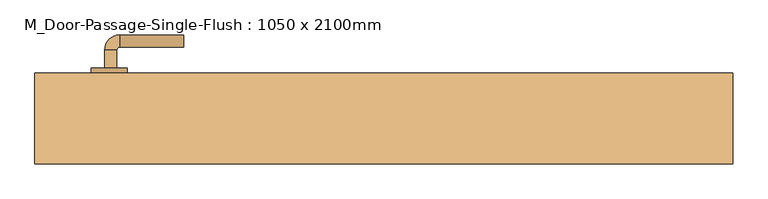
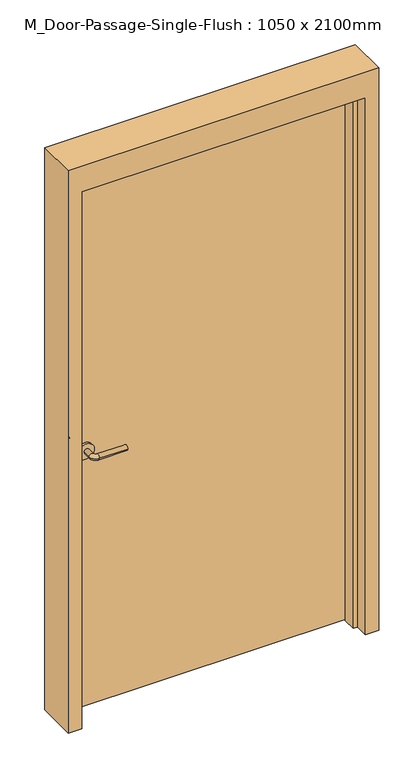
"""IFC4 building model written with IfcOpenShell, lengths in millimetres: door geometry, M_Door-Passage-Single-Flush : 1050 x 2100mm."""

import ifcopenshell
import ifcopenshell.guid

model = None  # the IFC model being written
_history = None  # IfcOwnerHistory: only IFC2X3 demands one
_inside = {}  # id of a spatial element -> (the spatial element, [elements in it])
_under = {}  # id of a project, library or spatial element -> (it, [spatial elements below it])
_declared = {}  # id of a project -> (the project, [libraries it declares])
_typed = {}  # id of a type object -> (the type object, [elements of that type])
_made_of = {}  # id of a material, layer set ... -> (it, [elements and type objects made of it])


def new_model(schema):
    """Start an empty IFC model of exactly this schema.

    Asked for "IFC4X3", IfcOpenShell would pick the latest addendum, in which some entities
    have other attributes; the version numbers below select the first issue.
    IFC2X3 requires an IfcOwnerHistory on every rooted entity: one is made here for all.
    """
    global model, _history
    if schema == "IFC4X3":
        model = ifcopenshell.file(schema_version=(4, 3, 0, 0))
    else:
        model = ifcopenshell.file(schema=schema)
    _inside.clear()
    _under.clear()
    _declared.clear()
    _typed.clear()
    _made_of.clear()
    _history = None
    if model.schema == "IFC2X3":
        org = make("IfcOrganization", Name="unknown")
        user = make(
            "IfcPersonAndOrganization",
            ThePerson=make("IfcPerson", FamilyName="unknown"),
            TheOrganization=org,
        )
        app = make(
            "IfcApplication",
            ApplicationDeveloper=org,
            Version="unknown",
            ApplicationFullName="unknown",
            ApplicationIdentifier="unknown",
        )
        _history = make(
            "IfcOwnerHistory",
            OwningUser=user,
            OwningApplication=app,
            ChangeAction="ADDED",
            CreationDate=0,
        )
    return model


def make(cls, **values):
    """One entity of the class cls with the attributes given. An attribute that is None is left unset."""
    return model.create_entity(
        cls, **{name: value for name, value in values.items() if value is not None}
    )


def rooted(cls, **values):
    """An entity with a GlobalId (a new one), such as an element, a storey or a relation."""
    return make(cls, GlobalId=ifcopenshell.guid.new(), OwnerHistory=_history, **values)


def si_unit(unit_type, name, prefix=None):
    """IfcSIUnit, for example si_unit("LENGTHUNIT", "METRE", prefix="MILLI")."""
    return make("IfcSIUnit", UnitType=unit_type, Prefix=prefix, Name=name)


def assignment(units):
    """IfcUnitAssignment: the units of a project."""
    return None if units is None else make("IfcUnitAssignment", Units=units)


def point(xyz):
    """IfcCartesianPoint."""
    return None if xyz is None else make("IfcCartesianPoint", Coordinates=xyz)


def direction(xyz):
    """IfcDirection."""
    return None if xyz is None else make("IfcDirection", DirectionRatios=xyz)


def frame(location, z_axis=None, x_axis=None):
    """IfcAxis2Placement3D, a coordinate frame: its origin and axes. An axis left out is left unset."""
    return make(
        "IfcAxis2Placement3D",
        Location=point(location),
        Axis=direction(z_axis),
        RefDirection=direction(x_axis),
    )


def frame_2d(location, x_axis=None):
    """IfcAxis2Placement2D, a coordinate frame in the plane: its origin and x axis."""
    return make(
        "IfcAxis2Placement2D", Location=point(location), RefDirection=direction(x_axis)
    )


def origin():
    """The frame at (0, 0, 0) with its axes left unset."""
    return frame((0.0, 0.0, 0.0))


def origin_with_axes():
    """The frame at (0, 0, 0) with the z axis (0, 0, 1) and the x axis (1, 0, 0) written out."""
    return frame((0.0, 0.0, 0.0), z_axis=(0.0, 0.0, 1.0), x_axis=(1.0, 0.0, 0.0))


def place(relative_to, where):
    """IfcLocalPlacement: puts the frame where relative to a parent placement (None: the world)."""
    return make(
        "IfcLocalPlacement", PlacementRelTo=relative_to, RelativePlacement=where
    )


def context(
    kind, dimensions, precision=None, world=None, true_north=None, identifier=None
):
    """IfcGeometricRepresentationContext, for example the 3D "Model" context."""
    return make(
        "IfcGeometricRepresentationContext",
        ContextIdentifier=identifier,
        ContextType=kind,
        CoordinateSpaceDimension=dimensions,
        Precision=precision,
        WorldCoordinateSystem=world,
        TrueNorth=true_north,
    )


def project(units=None, contexts=None):
    """IfcProject with its units and contexts."""
    return rooted(
        "IfcProject",
        Name="project",
        RepresentationContexts=contexts,
        UnitsInContext=assignment(units),
    )


def spatial(cls, under=None, at=None, **own):
    """A site, building, storey or space (cls), placed at a placement, below another one or the project."""
    s = rooted(cls, ObjectPlacement=at, **own)
    if under is not None:
        _under.setdefault(under.id(), (under, []))[1].append(s)
    return s


def polyline(points):
    """IfcPolyline through the points."""
    return make("IfcPolyline", Points=[point(p) for p in points])


def circle_curve(where, radius):
    """IfcCircle in the frame where."""
    return make("IfcCircle", Position=where, Radius=radius)


def ellipse_curve(where, semi_axis1, semi_axis2):
    """IfcEllipse in the frame where."""
    return make(
        "IfcEllipse", Position=where, SemiAxis1=semi_axis1, SemiAxis2=semi_axis2
    )


def trimmed(basis, trim1, trim2, sense, master):
    """IfcTrimmedCurve: the piece of a basis curve between two trims."""
    return make(
        "IfcTrimmedCurve",
        BasisCurve=basis,
        Trim1=trim1,
        Trim2=trim2,
        SenseAgreement=sense,
        MasterRepresentation=master,
    )


def segment(curve, same_sense, transition):
    """IfcCompositeCurveSegment."""
    return make(
        "IfcCompositeCurveSegment",
        Transition=transition,
        SameSense=same_sense,
        ParentCurve=curve,
    )


def composite_curve(segments, self_intersect=None):
    """IfcCompositeCurve: segments joined end to end."""
    return make("IfcCompositeCurve", Segments=segments, SelfIntersect=self_intersect)


def outline(outer, holes=None, kind="AREA"):
    """IfcArbitraryClosedProfileDef: a profile drawn as a closed curve; with holes, ...WithVoids."""
    if holes is None:
        return make("IfcArbitraryClosedProfileDef", ProfileType=kind, OuterCurve=outer)
    return make(
        "IfcArbitraryProfileDefWithVoids",
        ProfileType=kind,
        OuterCurve=outer,
        InnerCurves=holes,
    )


def extrude(swept, where, along, depth):
    """IfcExtrudedAreaSolid: the profile swept, set in the frame where, extruded along a direction by depth."""
    return make(
        "IfcExtrudedAreaSolid",
        SweptArea=swept,
        Position=where,
        ExtrudedDirection=direction(along),
        Depth=depth,
    )


def faces_of(points, faces, orient=None, outer=None):
    """IfcFace entities. A face is a list of loops; a loop is a list of indices into points, from 0.

    orient and outer hold one flag for each loop. By default every Orientation is true, the
    first loop of a face is its IfcFaceOuterBound and the others are IfcFaceBound.
    """
    made = []
    for i, loops in enumerate(faces):
        bounds = []
        for j, loop in enumerate(loops):
            is_outer = j == 0 if outer is None else outer[i][j]
            bounds.append(
                make(
                    "IfcFaceOuterBound" if is_outer else "IfcFaceBound",
                    Bound=make("IfcPolyLoop", Polygon=[points[k] for k in loop]),
                    Orientation=True if orient is None else orient[i][j],
                )
            )
        made.append(make("IfcFace", Bounds=bounds))
    return made


def faceted_brep(points, faces, orient=None, outer=None, voids=None):
    """IfcFacetedBrep: a solid bounded by flat faces; with voids (closed shells), ...WithVoids."""
    shared = [point(p) for p in points]
    hull = make("IfcClosedShell", CfsFaces=faces_of(shared, faces, orient, outer))
    if voids is None:
        return make("IfcFacetedBrep", Outer=hull)
    return make(
        "IfcFacetedBrepWithVoids",
        Outer=hull,
        Voids=[
            make(cls, CfsFaces=faces_of(shared, fs, o, b)) for cls, fs, o, b in voids
        ],
    )


def shape(context_of_items, identifier, shape_type, items):
    """IfcShapeRepresentation: the items that make up one representation, for example the "Body"."""
    return make(
        "IfcShapeRepresentation",
        ContextOfItems=context_of_items,
        RepresentationIdentifier=identifier,
        RepresentationType=shape_type,
        Items=items,
    )


def source(mapping_origin, context_of_items, identifier, shape_type, items):
    """IfcRepresentationMap: a shape defined once, which mapped items show again and again."""
    return make(
        "IfcRepresentationMap",
        MappingOrigin=mapping_origin,
        MappedRepresentation=shape(context_of_items, identifier, shape_type, items),
    )


def transform(
    local_origin,
    x_axis=None,
    y_axis=None,
    z_axis=None,
    scale=None,
    scale2=None,
    scale3=None,
    uniform=True,
):
    """IfcCartesianTransformationOperator3D, or its non-uniform kind. x_axis, y_axis, z_axis: its Axis1, 2, 3."""
    if uniform:
        return make(
            "IfcCartesianTransformationOperator3D",
            Axis1=direction(x_axis),
            Axis2=direction(y_axis),
            LocalOrigin=point(local_origin),
            Scale=scale,
            Axis3=direction(z_axis),
        )
    return make(
        "IfcCartesianTransformationOperator3DnonUniform",
        Axis1=direction(x_axis),
        Axis2=direction(y_axis),
        LocalOrigin=point(local_origin),
        Scale=scale,
        Axis3=direction(z_axis),
        Scale2=scale2,
        Scale3=scale3,
    )


def mapped(mapping_source, mapping_target):
    """IfcMappedItem: shows the shape of a source again, moved by a transform."""
    return make(
        "IfcMappedItem", MappingSource=mapping_source, MappingTarget=mapping_target
    )


def made_of(thing, what):
    """Note that an element or type object is made of a material, layer set ...; save() writes the relation."""
    if what is not None:
        _made_of.setdefault(what.id(), (what, []))[1].append(thing)
    return thing


def element(
    cls,
    number,
    at=None,
    inside=None,
    cuts=None,
    type_object=None,
    material=None,
    context=None,
    identifier="Body",
    shape_type=None,
    held_by="IfcProductDefinitionShape",
    body=None,
    shapes=None,
    **own,
):
    """One element of the class cls, such as IfcWall. Its Tag is "e" and its number.

    at: its placement. inside: the storey or other place that contains it. cuts: it is an
    opening in that element (IfcRelVoidsElement). A single representation is given by context,
    identifier, shape_type and body (its items); several are given by shapes. held_by: the class
    of the entity that holds the representations. save() writes the other relations.
    """
    e = rooted(cls, Tag="e%d" % number, ObjectPlacement=at, **own)
    if body is not None:
        shapes = [shape(context, identifier, shape_type, body)]
    if shapes is not None:
        e.Representation = make(held_by, Representations=shapes)
    if inside is not None:
        _inside.setdefault(inside.id(), (inside, []))[1].append(e)
    if cuts is not None:
        rooted(
            "IfcRelVoidsElement", RelatingBuildingElement=cuts, RelatedOpeningElement=e
        )
    if type_object is not None:
        _typed.setdefault(type_object.id(), (type_object, []))[1].append(e)
    return made_of(e, material)


def aggregate(whole, parts):
    """IfcRelAggregates: a whole, such as a stair, and the parts it consists of."""
    return rooted("IfcRelAggregates", RelatingObject=whole, RelatedObjects=parts)


def save(model, path):
    """Write the relations noted so far, then the file.

    IfcRelAggregates (storeys below a building ...), IfcRelContainedInSpatialStructure (elements
    in a storey), IfcRelDefinesByType, IfcRelAssociatesMaterial and IfcRelDeclares: one each for
    every whole, place, type object, material and project.
    """
    for whole, parts in _under.values():
        aggregate(whole, parts)
    for where, things in _inside.values():
        rooted(
            "IfcRelContainedInSpatialStructure",
            RelatedElements=things,
            RelatingStructure=where,
        )
    for kind, things in _typed.values():
        rooted("IfcRelDefinesByType", RelatedObjects=things, RelatingType=kind)
    for what, things in _made_of.values():
        rooted("IfcRelAssociatesMaterial", RelatedObjects=things, RelatingMaterial=what)
    for by, libraries in _declared.values():
        rooted("IfcRelDeclares", RelatingContext=by, RelatedDefinitions=libraries)
    model.write(path)


def plane_surface(at):
    """IfcPlane: the flat surface through the origin of the frame at, square to its z axis."""
    return make("IfcPlane", Position=at)


def cylinder_surface(at, radius):
    """IfcCylindricalSurface: all points at the distance radius from the z axis of the frame at."""
    return make("IfcCylindricalSurface", Position=at, Radius=radius)


def revolved_surface(curve, axis_point, axis_direction):
    """IfcSurfaceOfRevolution: the curve turned about the line through axis_point along axis_direction."""
    return make(
        "IfcSurfaceOfRevolution",
        SweptCurve=make("IfcArbitraryOpenProfileDef", ProfileType="CURVE", Curve=curve),
        AxisPosition=make("IfcAxis1Placement", Location=point(axis_point), Axis=direction(axis_direction)),
    )


def advanced_brep(points, edges, surfaces, faces):
    """IfcAdvancedBrep: a solid bounded by faces that lie on surfaces and meet in shared edges.

    An edge is (start, end): straight between two places in points (the first is 0);
    or (start, end, curve); or (start, end, curve, False) where it runs against its curve.
    A face is (place in surfaces, loops), or (place, loops, False) where it looks against
    its surface's normal. A loop lists edges by number (the first is 1), with a minus sign
    where the edge is run from its end to its start. The first loop is the outer one.
    """
    corners = [point(p) for p in points]
    vertices = [make("IfcVertexPoint", VertexGeometry=c) for c in corners]
    made = []
    for start, end, *more in edges:
        made.append(
            make(
                "IfcEdgeCurve",
                EdgeStart=vertices[start],
                EdgeEnd=vertices[end],
                EdgeGeometry=more[0] if more else make("IfcPolyline", Points=[corners[start], corners[end]]),
                SameSense=more[1] if len(more) > 1 else True,
            )
        )
    hull = []
    for where, loops, *sense in faces:
        bounds = []
        for j, loop in enumerate(loops):
            ring = [make("IfcOrientedEdge", EdgeElement=made[abs(k) - 1], Orientation=k > 0) for k in loop]
            bounds.append(
                make(
                    "IfcFaceOuterBound" if j == 0 else "IfcFaceBound",
                    Bound=make("IfcEdgeLoop", EdgeList=ring),
                    Orientation=True,
                )
            )
        hull.append(make("IfcAdvancedFace", Bounds=bounds, FaceSurface=surfaces[where], SameSense=sense[0] if sense else True))
    return make("IfcAdvancedBrep", Outer=make("IfcClosedShell", CfsFaces=hull))


def m_door_passage_single_flush_1050_x_2100mm_780507da(model_context):
    return source(origin(), model_context, "Body", "SolidModel", [
        advanced_brep(
        [(-459.990625, 78.35, 1000.0), (-439.990625, 78.35, 1000.0), (-439.990625, 48.35, 1000.0), (-459.990625, 48.35, 1000.0), (-434.990625, 43.35, 1000.0), (-434.990625, 23.35, 1000.0), (-329.990625, 23.35, 1000.0), (-329.990625, 43.35, 1000.0)],
        [
            (0, 1, circle_curve(frame((-449.990625, 78.35, 1000.0), z_axis=(0.0, 1.0, 0.0), x_axis=(1.0, 0.0, 0.0)), 10.0)),
            (1, 0, circle_curve(frame((-449.990625, 78.35, 1000.0), z_axis=(0.0, 1.0, 0.0), x_axis=(1.0, 0.0, 0.0)), 10.0)),
            (1, 2),
            (2, 3, circle_curve(frame((-449.990625, 48.35, 1000.0), z_axis=(0.0, 1.0, 0.0), x_axis=(1.0, 0.0, 0.0)), 10.0)),
            (3, 0),
            (3, 2, circle_curve(frame((-449.990625, 48.35, 1000.0), z_axis=(0.0, 1.0, 0.0), x_axis=(1.0, 0.0, 0.0)), 10.0)),
            (4, 5, circle_curve(frame((-434.990625, 33.35, 1000.0), z_axis=(-1.0, 0.0, 0.0), x_axis=(0.0, 1.0, 0.0)), 10.0)),
            (5, 3, circle_curve(frame((-434.990625, 48.35, 1000.0), z_axis=(0.0, 0.0, -1.0), x_axis=(-1.0, 0.0, 0.0)), 25.0)),
            (2, 4, circle_curve(frame((-434.990625, 48.35, 1000.0), z_axis=(0.0, 0.0, 1.0), x_axis=(-1.0, 0.0, 0.0)), 5.0)),
            (5, 4, circle_curve(frame((-434.990625, 33.35, 1000.0), z_axis=(-1.0, 0.0, 0.0), x_axis=(0.0, 1.0, 0.0)), 10.0)),
            (6, 7, circle_curve(frame((-329.990625, 33.35, 1000.0), z_axis=(1.0, 0.0, 0.0), x_axis=(0.0, 1.0, 0.0)), 10.0)),
            (7, 6, circle_curve(frame((-329.990625, 33.35, 1000.0), z_axis=(1.0, 0.0, 0.0), x_axis=(0.0, 1.0, 0.0)), 10.0)),
            (4, 7),
            (6, 5),
        ],
        [
            plane_surface(frame((-449.990625, 78.35, 1000.0), z_axis=(0.0, 1.0, 0.0), x_axis=(0.0, 0.0, 1.0))),
            cylinder_surface(frame((-449.990625, 78.35, 1000.0), z_axis=(0.0, 1.0, 0.0), x_axis=(1.0, 0.0, 0.0)), 10.0),
            revolved_surface(trimmed(ellipse_curve(frame((-449.990625, 48.35, 1000.0), z_axis=(0.0, -1.0, 0.0), x_axis=(1.0, 0.0, 0.0)), 10.0, 10.0), [point((-459.990625, 48.35, 1000.0))], [point((-439.990625, 48.35, 1000.0))], True, "CARTESIAN"), (-434.990625, 48.35, 1000.0), (0.0, 0.0, -1.0)),
            revolved_surface(trimmed(ellipse_curve(frame((-449.990625, 48.35, 1000.0), z_axis=(0.0, -1.0, 0.0), x_axis=(1.0, 0.0, 0.0)), 10.0, 10.0), [point((-439.990625, 48.35, 1000.0))], [point((-459.990625, 48.35, 1000.0))], True, "CARTESIAN"), (-434.990625, 48.35, 1000.0), (0.0, 0.0, -1.0)),
            plane_surface(frame((-329.990625, 33.35, 1000.0), z_axis=(1.0, 0.0, 0.0), x_axis=(0.0, 0.0, 1.0))),
            cylinder_surface(frame((-434.990625, 33.35, 1000.0), z_axis=(-1.0, 0.0, 0.0), x_axis=(0.0, 1.0, 0.0)), 10.0),
        ],
        [
            (0, [[1, 2]]),
            (1, [[3, 4, 5, -2]]),
            (1, [[-5, 6, -3, -1]]),
            (2, [[7, 8, -4, 9]]),
            (3, [[10, -9, -6, -8]]),
            (4, [[11, 12]]),
            (5, [[13, -11, 14, -7]]),
            (5, [[-14, -12, -13, -10]]),
        ],
    ),
        extrude(outline(composite_curve([segment(trimmed(circle_curve(frame_2d((1000.0, -452.490625)), 30.0), [point((1000.0, -482.490625))], [point((1000.0, -422.490625))], False, "CARTESIAN"), True, "CONTINUOUS"), segment(trimmed(circle_curve(frame_2d((1000.0, -452.490625)), 30.0), [point((1000.0, -422.490625))], [point((1000.0, -482.490625))], False, "CARTESIAN"), True, "CONTINUOUS")], self_intersect=False)), frame((0.0, 78.35, 0.0), z_axis=(0.0, 1.0, 0.0), x_axis=(0.0, 0.0, 1.0)), (0.0, 0.0, 1.0), 8.0),
        advanced_brep(
        [(-459.990625, 139.35, 1000.0), (-439.990625, 139.35, 1000.0), (-459.990625, 169.35, 1000.0), (-439.990625, 169.35, 1000.0), (-434.990625, 174.35, 1000.0), (-434.990625, 194.35, 1000.0), (-329.990625, 194.35, 1000.0), (-329.990625, 174.35, 1000.0)],
        [
            (0, 1, circle_curve(frame((-449.990625, 139.35, 1000.0), z_axis=(0.0, -1.0, 0.0), x_axis=(1.0, 0.0, 0.0)), 10.0)),
            (1, 0, circle_curve(frame((-449.990625, 139.35, 1000.0), z_axis=(0.0, -1.0, 0.0), x_axis=(1.0, 0.0, 0.0)), 10.0)),
            (0, 2),
            (2, 3, circle_curve(frame((-449.990625, 169.35, 1000.0), z_axis=(0.0, -1.0, 0.0), x_axis=(1.0, 0.0, 0.0)), 10.0)),
            (3, 1),
            (3, 2, circle_curve(frame((-449.990625, 169.35, 1000.0), z_axis=(0.0, -1.0, 0.0), x_axis=(1.0, 0.0, 0.0)), 10.0)),
            (4, 3, circle_curve(frame((-434.990625, 169.35, 1000.0), z_axis=(0.0, 0.0, 1.0), x_axis=(-1.0, 0.0, 0.0)), 5.0)),
            (2, 5, circle_curve(frame((-434.990625, 169.35, 1000.0), z_axis=(0.0, 0.0, -1.0), x_axis=(-1.0, 0.0, 0.0)), 25.0)),
            (5, 4, circle_curve(frame((-434.990625, 184.35, 1000.0), z_axis=(-1.0, 0.0, 0.0), x_axis=(0.0, -1.0, 0.0)), 10.0)),
            (4, 5, circle_curve(frame((-434.990625, 184.35, 1000.0), z_axis=(-1.0, 0.0, 0.0), x_axis=(0.0, -1.0, 0.0)), 10.0)),
            (6, 7, circle_curve(frame((-329.990625, 184.35, 1000.0), z_axis=(1.0, 0.0, 0.0), x_axis=(0.0, -1.0, 0.0)), 10.0)),
            (7, 6, circle_curve(frame((-329.990625, 184.35, 1000.0), z_axis=(1.0, 0.0, 0.0), x_axis=(0.0, -1.0, 0.0)), 10.0)),
            (5, 6),
            (7, 4),
        ],
        [
            plane_surface(frame((-449.990625, 139.35, 1000.0), z_axis=(0.0, -1.0, 0.0), x_axis=(0.0, 0.0, 1.0))),
            cylinder_surface(frame((-449.990625, 139.35, 1000.0), z_axis=(0.0, -1.0, 0.0), x_axis=(1.0, 0.0, 0.0)), 10.0),
            revolved_surface(trimmed(ellipse_curve(frame((-449.990625, 169.35, 1000.0), z_axis=(0.0, -1.0, 0.0), x_axis=(1.0, 0.0, 0.0)), 10.0, 10.0), [point((-459.990625, 169.35, 1000.0))], [point((-439.990625, 169.35, 1000.0))], True, "CARTESIAN"), (-434.990625, 169.35, 1000.0), (0.0, 0.0, -1.0)),
            revolved_surface(trimmed(ellipse_curve(frame((-449.990625, 169.35, 1000.0), z_axis=(0.0, -1.0, 0.0), x_axis=(1.0, 0.0, 0.0)), 10.0, 10.0), [point((-439.990625, 169.35, 1000.0))], [point((-459.990625, 169.35, 1000.0))], True, "CARTESIAN"), (-434.990625, 169.35, 1000.0), (0.0, 0.0, -1.0)),
            plane_surface(frame((-329.990625, 184.35, 1000.0), z_axis=(1.0, 0.0, 0.0), x_axis=(0.0, 0.0, 1.0))),
            cylinder_surface(frame((-434.990625, 184.35, 1000.0), z_axis=(-1.0, 0.0, 0.0), x_axis=(0.0, -1.0, 0.0)), 10.0),
        ],
        [
            (0, [[1, 2]]),
            (1, [[-1, 3, 4, 5]]),
            (1, [[-2, -5, 6, -3]]),
            (2, [[7, -4, 8, 9]]),
            (3, [[-8, -6, -7, 10]]),
            (4, [[11, 12]]),
            (5, [[-9, 13, -12, 14]]),
            (5, [[-10, -14, -11, -13]]),
        ],
    ),
        extrude(outline(composite_curve([segment(trimmed(circle_curve(frame_2d((1000.0, -452.490625)), 30.0), [point((1000.0, -482.490625))], [point((1000.0, -422.490625))], False, "CARTESIAN"), True, "CONTINUOUS"), segment(trimmed(circle_curve(frame_2d((1000.0, -452.490625)), 30.0), [point((1000.0, -422.490625))], [point((1000.0, -482.490625))], False, "CARTESIAN"), True, "CONTINUOUS")], self_intersect=False)), frame((0.0, 131.35, 0.0), z_axis=(0.0, 1.0, 0.0), x_axis=(0.0, 0.0, 1.0)), (0.0, 0.0, 1.0), 8.0),
        faceted_brep([(525.0, 81.5875, 0.0), (525.0, 131.35, 0.0), (575.0, 131.35, 0.0), (575.0, -18.65, 0.0), (525.0, -18.65, 0.0), (525.0, 30.5625, 0.0), (509.125, 30.5625, 0.0), (509.125, 81.5875, 0.0), (525.0, 81.5875, 2100.0), (525.0, 131.35, 2100.0), (-525.0, 131.35, 2100.0), (-525.0, 131.35, 0.0), (-575.0, 131.35, 0.0), (-575.0, 131.35, 2200.0), (575.0, 131.35, 2200.0), (575.0, -18.65, 2200.0), (-575.0, -18.65, 2200.0), (-575.0, -18.65, 0.0), (-525.0, -18.65, 0.0), (-525.0, -18.65, 2100.0), (525.0, -18.65, 2100.0), (525.0, 30.5625, 2100.0), (-525.0, 30.5625, 2100.0), (-525.0, 30.5625, 0.0), (-509.125, 30.5625, 0.0), (-509.125, 30.5625, 2084.125), (509.125, 30.5625, 2084.125), (509.125, 81.5875, 2084.125), (-509.125, 81.5875, 2084.125), (-509.125, 81.5875, 0.0), (-525.0, 81.5875, 0.0), (-525.0, 81.5875, 2100.0)], [[[0, 1, 2, 3, 4, 5, 6, 7]], [[1, 0, 8, 9]], [[2, 1, 9, 10, 11, 12, 13, 14]], [[3, 2, 14, 15]], [[4, 3, 15, 16, 17, 18, 19, 20]], [[5, 4, 20, 21]], [[6, 5, 21, 22, 23, 24, 25, 26]], [[7, 6, 26, 27]], [[0, 7, 27, 28, 29, 30, 31, 8]], [[9, 8, 31, 10]], [[20, 19, 22, 21]], [[26, 25, 28, 27]], [[12, 11, 30, 29, 24, 23, 18, 17]], [[11, 10, 31, 30]], [[13, 12, 17, 16]], [[19, 18, 23, 22]], [[25, 24, 29, 28]], [[15, 14, 13, 16]]]),
        extrude(outline(polyline([(525.0, 86.35), (-525.0, 86.35), (-525.0, 131.35), (525.0, 131.35), (525.0, 86.35)])), origin_with_axes(), (0.0, 0.0, 1.0), 2100.0),
    ])


if __name__ == "__main__":
    model = new_model("IFC4")
    model_context = context("Model", 3, world=origin())
    ifc_project = project(units=[si_unit("LENGTHUNIT", "METRE", prefix="MILLI")], contexts=[model_context])
    site = spatial("IfcSite", under=ifc_project)
    building = spatial("IfcBuilding", under=site)
    placement = place(None, origin())
    m_door_passage_single_flush_1050_x_2100mm_shape = m_door_passage_single_flush_1050_x_2100mm_780507da(model_context)
    element("IfcDoor", 1, ObjectType="M_Door-Passage-Single-Flush : 1050 x 2100mm", at=placement, inside=building, context=model_context, shape_type="MappedRepresentation", body=[
        mapped(m_door_passage_single_flush_1050_x_2100mm_shape, transform((0.0, 0.0, 0.0), x_axis=(1.0, 0.0, 0.0), y_axis=(0.0, 1.0, 0.0), z_axis=(0.0, 0.0, 1.0))),
    ])
    save(model, "model.ifc")

# Revit data of these elements
# Type "M_Door-Passage-Single-Flush : 1050 x 2100mm"
#   Type Mark = "39"
#   Assembly Code = "B2030200"
#   Analytic Construction = "Wooden"
#   Thickness = 45 mm
#   Thermal Resistance (R) = 0.455703 (m²·K)/W
#   Swing Angle [instance default] = 90.00°
#   Strike Height = 1000 mm
#   Rough Width [instance default] = 1150 mm
#   Rough Height [instance default] = 2200 mm
#   MF Opening Height [instance default] = 100 mm
#   MF Opening Width [instance default] = 100 mm
#   Inset Calculate [instance default] = 105 mm
#   Masonry Inset [instance default] = 25 mm
#   Height = 2100 mm
#   Width = 1050 mm
#   Heat Transfer Coefficient (U) = 2.19465 W/(m²·K)
#   Masonry Frame Depth = 150 mm
#   Masonry Frame [instance default] = yes
#   Function = 1
#   Dry Wall Frame [instance default] = no
#   Panel Material = Wood - Birch
#   Frame Material = Metal - Paint Finish - Grey
#   Door Handle Material = Aluminum
#   Visual Light Transmittance = 0
#   Solar Heat Gain Coefficient = 0
#   Wall Closure = (empty or 0)
# Element 1 (IfcDoor, "M_Door-Passage-Single-Flush : 1050 x 2100mm")
#   Materials on its faces: "Aluminum", "Metal - Paint Finish - Grey", "Wood - Birch"
# Materials
#   "Wood - Birch": class "Wood", colour RGB 166 116 52, transparency 0, Cost = 0
#   "Metal - Paint Finish - Grey": class "Paint", colour RGB 104 104 104, transparency 0, Cost = 0
#   "Aluminum": class "Metal", colour RGB 244 244 244, transparency 0, Description = "Aluminum 6061", Cost = 0
